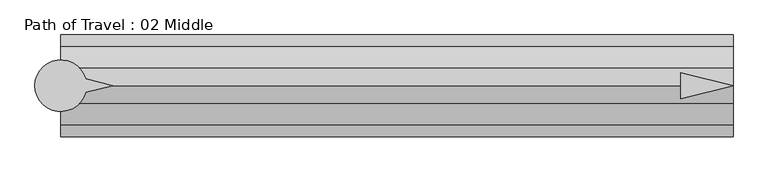
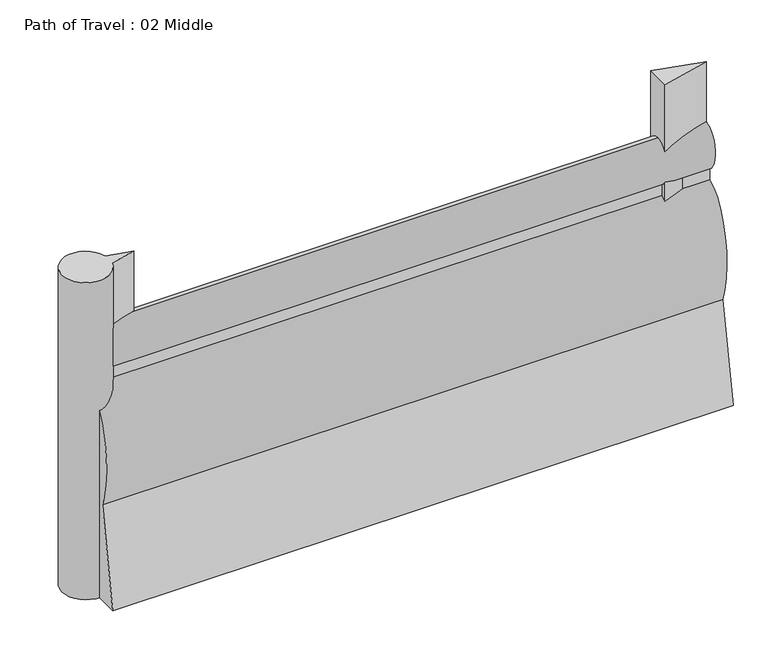
"""IFC4 building model written with IfcOpenShell, lengths in millimetres: proxy geometry, Path of Travel : 02 Middle."""

from ifc_helpers import new_model, si_unit, point, frame, frame_2d, origin, origin_with_axes, place, context, project, spatial, polyline, circle_curve, ellipse_curve, trimmed, segment, composite_curve, outline, extrude, source, transform, mapped, element, save
from ifc_brep_helpers import plane_surface, extruded_surface, advanced_brep


def path_of_travel_02_middle_53b68d80(model_context):
    return source(origin(), model_context, "Body", "SolidModel", [
        advanced_brep(
        [(227.5554837, 0.0, 1727.2), (227.5554837, 42.9018657, 1436.6534209), (227.5554837, 42.9018657, 1363.4763406), (227.5554837, 184.1186263, 643.4144547), (227.5554837, 297.5699544, 0.0), (227.5554837, 145.6574193, 0.0), (227.5554837, 0.0, 584.2), (227.5554837, -145.6574193, 0.0), (227.5554837, -297.5699544, 0.0), (227.5554837, -184.1186263, 643.4144547), (227.5554837, -42.9018657, 1363.4763406), (227.5554837, -42.9018657, 1436.6534209), (4165.3302308, 0.0, 1727.2), (4165.3302308, -42.9018657, 1436.6534209), (4165.3302308, -42.9018657, 1363.4763406), (4165.3302308, -184.1186263, 643.4144547), (4165.3302308, -297.5699544, 0.0), (4165.3302308, -145.6574193, 0.0), (4165.3302308, 0.0, 584.2), (4165.3302308, 145.6574193, 0.0), (4165.3302308, 297.5699544, 0.0), (4165.3302308, 184.1186263, 643.4144547), (4165.3302308, 42.9018657, 1363.4763406), (4165.3302308, 42.9018657, 1436.6534209)],
        [
            (0, 1, ellipse_curve(frame((227.5554837, 0.0, 1574.8), z_axis=(-1.0, 0.0, 0.0), x_axis=(0.0, 0.0, 1.0)), 152.4, 101.6)),
            (1, 2),
            (2, 3, ellipse_curve(frame((227.5554837, 0.0, 914.4), z_axis=(-1.0, 0.0, 0.0), x_axis=(0.0, 0.0, -1.0)), 457.2, 228.6)),
            (3, 4),
            (4, 5),
            (5, 6),
            (6, 7),
            (7, 8),
            (8, 9),
            (9, 10, ellipse_curve(frame((227.5554837, 0.0, 914.4), z_axis=(-1.0, 0.0, 0.0), x_axis=(0.0, 0.0, -1.0)), 457.2, 228.6)),
            (10, 11),
            (11, 0, ellipse_curve(frame((227.5554837, 0.0, 1574.8), z_axis=(-1.0, 0.0, 0.0), x_axis=(0.0, 0.0, 1.0)), 152.4, 101.6)),
            (12, 13, ellipse_curve(frame((4165.3302308, 0.0, 1574.8), z_axis=(1.0, 0.0, 0.0), x_axis=(0.0, 0.0, 1.0)), 152.4, 101.6)),
            (13, 14),
            (14, 15, ellipse_curve(frame((4165.3302308, 0.0, 914.4), z_axis=(1.0, 0.0, 0.0), x_axis=(0.0, 0.0, -1.0)), 457.2, 228.6)),
            (15, 16),
            (16, 17),
            (17, 18),
            (18, 19),
            (19, 20),
            (20, 21),
            (21, 22, ellipse_curve(frame((4165.3302308, 0.0, 914.4), z_axis=(1.0, 0.0, 0.0), x_axis=(0.0, 0.0, -1.0)), 457.2, 228.6)),
            (22, 23),
            (23, 12, ellipse_curve(frame((4165.3302308, 0.0, 1574.8), z_axis=(1.0, 0.0, 0.0), x_axis=(0.0, 0.0, 1.0)), 152.4, 101.6)),
            (0, 12),
            (23, 1),
            (22, 2),
            (21, 3),
            (20, 4),
            (19, 5),
            (18, 6),
            (17, 7),
            (16, 8),
            (15, 9),
            (14, 10),
            (13, 11),
        ],
        [
            plane_surface(frame((227.5554837, 0.0, 0.0), z_axis=(-1.0, 0.0, 0.0), x_axis=(0.0, 0.0, 1.0))),
            plane_surface(frame((4165.3302308, 0.0, 0.0), z_axis=(1.0, 0.0, 0.0), x_axis=(0.0, 0.0, 1.0))),
            extruded_surface(trimmed(ellipse_curve(frame((4165.3302308, 0.0, 1574.8), z_axis=(-1.0, 0.0, 0.0), x_axis=(0.0, 0.0, 1.0)), 152.4, 101.6), [point((4165.3302308, 0.0, 1727.2))], [point((4165.3302308, 42.9018657, 1436.6534209))], True, "CARTESIAN"), (-3937.7747471000002, 0.0, 0.0), 3937.7747471000002),
            plane_surface(frame((227.5554837, 42.9018657, 1436.6534209), z_axis=(0.0, 1.0, 0.0), x_axis=(1.0, 0.0, 0.0))),
            extruded_surface(trimmed(ellipse_curve(frame((4165.3302308, 0.0, 914.4), z_axis=(-1.0, 0.0, 0.0), x_axis=(0.0, 0.0, -1.0)), 457.2, 228.6), [point((4165.3302308, 42.9018657, 1363.4763406))], [point((4165.3302308, 184.1186263, 643.4144547))], True, "CARTESIAN"), (-3937.7747471000002, 0.0, 0.0), 3937.7747471000002),
            plane_surface(frame((227.5554837, 184.1186263, 643.4144547), z_axis=(0.0, 0.9848077530122078, 0.1736481776669322), x_axis=(1.0, 0.0, 0.0))),
            plane_surface(frame((227.5554837, 297.5699544, 0.0), z_axis=(0.0, 0.0, -1.0), x_axis=(1.0, 0.0, 0.0))),
            plane_surface(frame((227.5554837, 145.6574193, 0.0), z_axis=(0.0, -0.9702957262760199, -0.2419218955995739), x_axis=(1.0, 0.0, 0.0))),
            plane_surface(frame((227.5554837, 0.0, 584.2), z_axis=(0.0, 0.9702957262759961, -0.24192189559966923), x_axis=(1.0, 0.0, 0.0))),
            plane_surface(frame((227.5554837, -145.6574193, 0.0), z_axis=(0.0, 0.0, -1.0), x_axis=(1.0, 0.0, 0.0))),
            plane_surface(frame((227.5554837, -297.5699544, 0.0), z_axis=(0.0, -0.984807753012208, 0.17364817766693066), x_axis=(1.0, 0.0, 0.0))),
            extruded_surface(trimmed(ellipse_curve(frame((4165.3302308, 0.0, 914.4), z_axis=(-1.0, 0.0, 0.0), x_axis=(0.0, 0.0, -1.0)), 457.2, 228.6), [point((4165.3302308, -184.1186263, 643.4144547))], [point((4165.3302308, -42.9018657, 1363.4763406))], True, "CARTESIAN"), (-3937.7747471000002, 0.0, 0.0), 3937.7747471000002),
            plane_surface(frame((227.5554837, -42.9018657, 1363.4763406), z_axis=(0.0, -1.0, 0.0), x_axis=(1.0, 0.0, 0.0))),
            extruded_surface(trimmed(ellipse_curve(frame((4165.3302308, 0.0, 1574.8), z_axis=(-1.0, 0.0, 0.0), x_axis=(0.0, 0.0, 1.0)), 152.4, 101.6), [point((4165.3302308, -42.9018657, 1436.6534209))], [point((4165.3302308, 0.0, 1727.2))], True, "CARTESIAN"), (-3937.7747471000002, 0.0, 0.0), 3937.7747471000002),
        ],
        [
            (0, [[1, 2, 3, 4, 5, 6, 7, 8, 9, 10, 11, 12]]),
            (1, [[13, 14, 15, 16, 17, 18, 19, 20, 21, 22, 23, 24]]),
            (2, [[-1, 25, -24, 26]]),
            (3, [[-2, -26, -23, 27]]),
            (4, [[-3, -27, -22, 28]]),
            (5, [[-4, -28, -21, 29]]),
            (6, [[-5, -29, -20, 30]]),
            (7, [[-6, -30, -19, 31]]),
            (8, [[-7, -31, -18, 32]]),
            (9, [[-8, -32, -17, 33]]),
            (10, [[-9, -33, -16, 34]]),
            (11, [[-10, -34, -15, 35]]),
            (12, [[-11, -35, -14, 36]]),
            (13, [[-12, -36, -13, -25]]),
        ],
    ),
        extrude(outline(polyline([(3859.3250843, 76.2006338), (4165.3302308, 0.0), (3859.3250843, -76.2006338), (3859.3250843, 76.2006338)])), origin_with_axes(), (0.0, 0.0, 1.0), 2129.5973753),
        extrude(outline(composite_curve([segment(polyline([(372.7837828, 39.4440225), (531.182385, 0.0), (372.7837828, -39.4440225)]), True, "CONTINUOUS"), segment(trimmed(circle_curve(frame_2d((227.2200886, 0.0)), 150.8131956), [point((372.7837828, -39.4440225))], [point((372.7837828, 39.4440225))], False, "CARTESIAN"), True, "CONTINUOUS")], self_intersect=False)), origin_with_axes(), (0.0, 0.0, 1.0), 2129.5973753),
    ])


if __name__ == "__main__":
    model = new_model("IFC4")
    model_context = context("Model", 3, world=origin())
    ifc_project = project(units=[si_unit("LENGTHUNIT", "METRE", prefix="MILLI")], contexts=[model_context])
    site = spatial("IfcSite", under=ifc_project)
    building = spatial("IfcBuilding", under=site)
    placement = place(None, origin())
    path_of_travel_02_middle_shape = path_of_travel_02_middle_53b68d80(model_context)
    element("IfcBuildingElementProxy", 1, Name="Path of Travel : 02 Middle", ObjectType="Path of Travel : 02 Middle", at=placement, inside=building, context=model_context, shape_type="MappedRepresentation", body=[
        mapped(path_of_travel_02_middle_shape, transform((0.0, 0.0, 0.0), x_axis=(1.0, 0.0, 0.0), y_axis=(0.0, 1.0, 0.0), z_axis=(0.0, 0.0, 1.0))),
    ])
    save(model, "model.ifc")

# Revit data of these elements
# Type "Path of Travel : 02 Middle"
#   Path of Egress [instance default] = 4' - 0"
#   built-in parameter 1001306 [instance default] = 4 (stored number, unit not read)
#   Dot at Start = no
#   Arrow in Middle = yes
#   Arrow at End = no
#   Egress Path = none
# Element 1 (IfcBuildingElementProxy, "Path of Travel : 02 Middle")
#   Path of Egress = 12' - 11.0305"
#   built-in parameter 1001306 = 12.9192 (stored number, unit not read)
